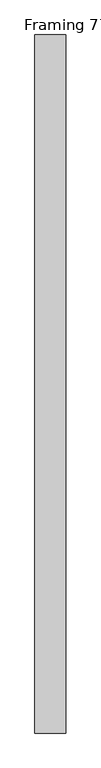
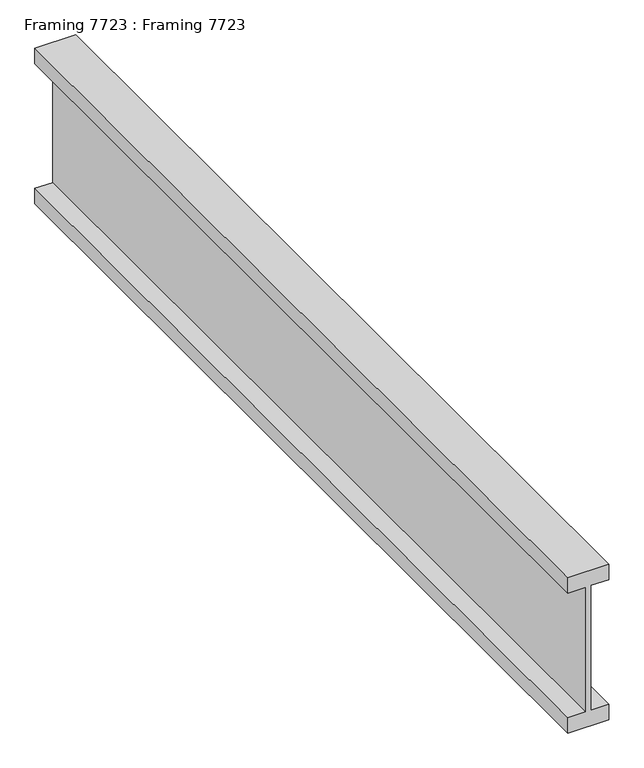
"""IFC4 building model written with IfcOpenShell, lengths in millimetres: proxy geometry, Framing 7723 : Framing 7723."""

from ifc_helpers import new_model, si_unit, frame, origin, place, context, project, spatial, polyline, outline, extrude, source, transform, mapped, element, save


def framing_7723_framing_7723_e96781f7(model_context):
    return source(origin(), model_context, "Body", "SweptSolid", [
        extrude(outline(polyline([(40077.771, 7689.895938), (39792.021, 7689.895938), (39792.021, 7651.002188), (39757.096, 7651.002188), (39757.096, 7739.902188), (39792.021, 7739.902188), (39792.021, 7701.008438), (40077.771, 7701.008438), (40077.771, 7739.902188), (40112.696, 7739.902188), (40112.696, 7651.002188), (40077.771, 7651.002188), (40077.771, 7689.895938)])), frame((0.0, -3747.9491938, 0.0), z_axis=(0.0, 1.0, 0.0), x_axis=(0.0, 0.0, 1.0)), (0.0, 0.0, 1.0), 2000.0),
    ])


if __name__ == "__main__":
    model = new_model("IFC4")
    model_context = context("Model", 3, world=origin())
    ifc_project = project(units=[si_unit("LENGTHUNIT", "METRE", prefix="MILLI")], contexts=[model_context])
    site = spatial("IfcSite", under=ifc_project)
    building = spatial("IfcBuilding", under=site)
    placement = place(None, origin())
    framing_7723_framing_7723_shape = framing_7723_framing_7723_e96781f7(model_context)
    element("IfcBuildingElementProxy", 1, Name="Framing 7723 : Framing 7723", ObjectType="Framing 7723 : Framing 7723", at=placement, inside=building, context=model_context, shape_type="MappedRepresentation", body=[
        mapped(framing_7723_framing_7723_shape, transform((0.0, 0.0, 0.0), x_axis=(1.0, 0.0, 0.0), y_axis=(0.0, 1.0, 0.0), z_axis=(0.0, 0.0, 1.0))),
    ])
    save(model, "model.ifc")

# Revit data of these elements
# Type "Framing 7723 : Framing 7723"
#   NameOverride = "Framing"
# Element 1 (IfcBuildingElementProxy, "Framing 7723 : Framing 7723")
#   Materials on its faces: "WOOD FRAMING (SEE STRUCT DWGS)"
# Materials
#   "WOOD FRAMING (SEE STRUCT DWGS)": class "Unassigned", colour RGB 224 188 168, transparency 0, Cost = 0
